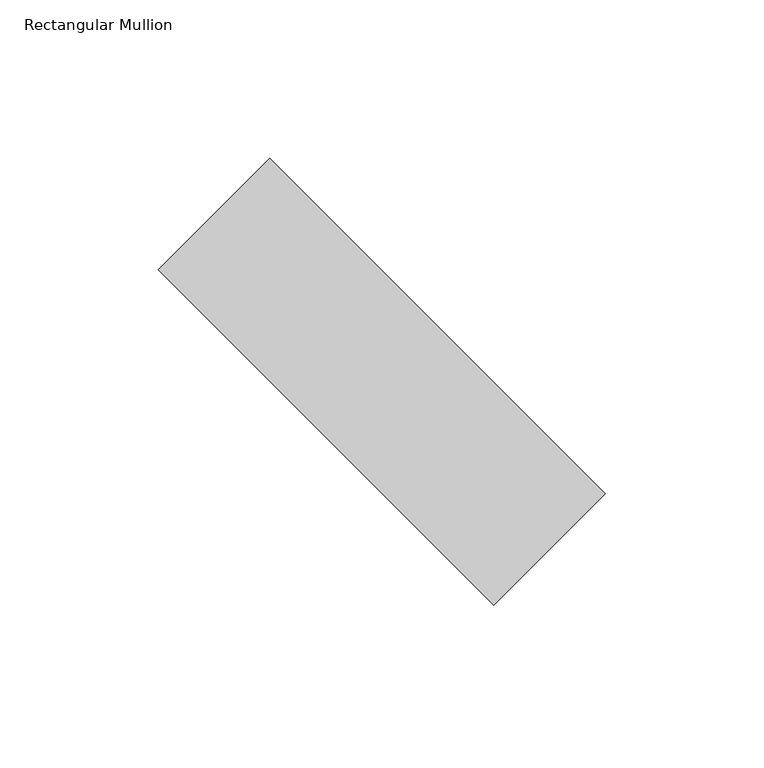
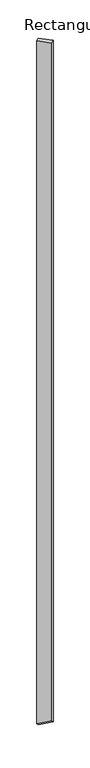
"""IFC4 building model written with IfcOpenShell, lengths in millimetres: member geometry, Rectangular Mullion : tilted mullions."""

from ifc_helpers import new_model, si_unit, origin, place, context, project, spatial, faceted_brep, source, transform, mapped, element, save


def rectangular_mullion_19cf8c27(model_context):
    return source(origin(), model_context, "Body", "Brep", [
        faceted_brep([(-35.3553391, 70.7106781, 0.0), (-70.7106781, 35.3553391, 0.0), (35.3553391, -70.7106781, 0.0), (70.7106781, -35.3553391, 0.0), (-35.3553391, 70.7106781, -8054.989187), (-70.7106781, 35.3553391, -8009.9256096), (35.3553391, -70.7106781, -7944.9374113), (70.7106781, -35.3553391, -7990.0009887)], [[[0, 1, 2, 3]], [[1, 0, 4, 5]], [[2, 1, 5, 6]], [[3, 2, 6, 7]], [[0, 3, 7, 4]], [[4, 7, 6, 5]]]),
    ])


if __name__ == "__main__":
    model = new_model("IFC4")
    model_context = context("Model", 3, world=origin())
    ifc_project = project(units=[si_unit("LENGTHUNIT", "METRE", prefix="MILLI")], contexts=[model_context])
    site = spatial("IfcSite", under=ifc_project)
    building = spatial("IfcBuilding", under=site)
    placement = place(None, origin())
    rectangular_mullion_shape = rectangular_mullion_19cf8c27(model_context)
    element("IfcMember", 1, ObjectType="Rectangular Mullion : tilted mullions", at=placement, inside=building, context=model_context, shape_type="MappedRepresentation", body=[
        mapped(rectangular_mullion_shape, transform((0.0, 0.0, 0.0), x_axis=(1.0, 0.0, 0.0), y_axis=(0.0, 1.0, 0.0), z_axis=(0.0, 0.0, 1.0))),
    ])
    save(model, "model.ifc")

# Revit data of these elements
# Type "Rectangular Mullion : tilted mullions"
#   built-in parameter 1007304 = 0.492126 (stored number, unit not read)
#   built-in parameter 1007301 = 0.082021 (stored number, unit not read)
#   built-in parameter 1007300 = 0.082021 (stored number, unit not read)
# Element 1 (IfcMember, "Rectangular Mullion : tilted mullions")
#   Materials on its faces: "Aluminum"
# Materials
#   "Aluminum": class "Metal", colour RGB 244 244 244, transparency 0, Description = "Aluminum 6061", Cost = 0
